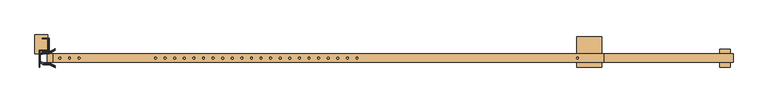
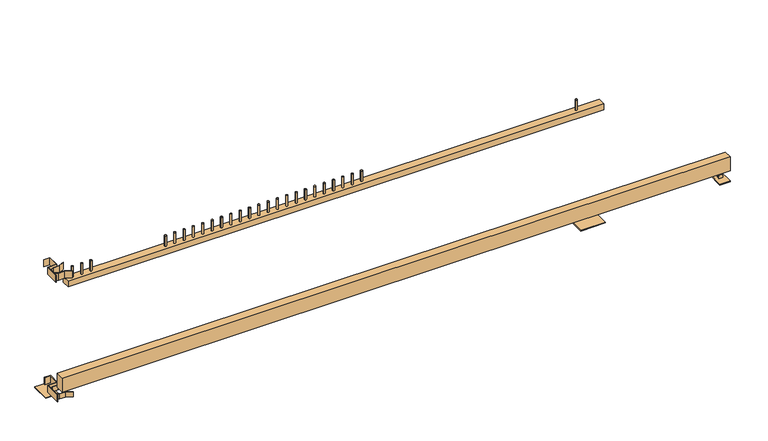
"""IFC4 building model written with IfcOpenShell, lengths in millimetres: door geometry, NLRS_90_DO_UN_schuifpoort met spijlen_gen_rsf : schuifpoort automatisch bxh 7000x1800-NP."""

from ifc_helpers import new_model, si_unit, point, frame, frame_2d, origin, origin_with_axes, place, context, project, spatial, polyline, circle_curve, trimmed, segment, composite_curve, outline, extrude, source, transform, mapped, element, save


def door_84a52a24(model_context):
    return source(origin(), model_context, "Body", "SweptSolid", [
        extrude(outline(composite_curve([segment(trimmed(circle_curve(frame_2d((-3115.5, 0.0)), 12.5), [point((-3103.0, 0.0))], [point((-3128.0, 0.0))], False, "CARTESIAN"), True, "CONTINUOUS"), segment(trimmed(circle_curve(frame_2d((-3115.5, 0.0)), 12.5), [point((-3128.0, 0.0))], [point((-3103.0, 0.0))], False, "CARTESIAN"), True, "CONTINUOUS")], self_intersect=False)), frame((0.0, 0.0, 1650.0), z_axis=(0.0, 0.0, 1.0), x_axis=(1.0, 0.0, 0.0)), (0.0, 0.0, 1.0), 150.0),
        extrude(outline(composite_curve([segment(trimmed(circle_curve(frame_2d((-3241.5, 0.0)), 12.5), [point((-3229.0, 0.0))], [point((-3254.0, 0.0))], False, "CARTESIAN"), True, "CONTINUOUS"), segment(trimmed(circle_curve(frame_2d((-3241.5, 0.0)), 12.5), [point((-3254.0, 0.0))], [point((-3229.0, 0.0))], False, "CARTESIAN"), True, "CONTINUOUS")], self_intersect=False)), frame((0.0, 0.0, 1650.0), z_axis=(0.0, 0.0, 1.0), x_axis=(1.0, 0.0, 0.0)), (0.0, 0.0, 1.0), 150.0),
        extrude(outline(composite_curve([segment(trimmed(circle_curve(frame_2d((-3367.5, 0.0)), 12.5), [point((-3355.0, 0.0))], [point((-3380.0, 0.0))], False, "CARTESIAN"), True, "CONTINUOUS"), segment(trimmed(circle_curve(frame_2d((-3367.5, 0.0)), 12.5), [point((-3380.0, 0.0))], [point((-3355.0, 0.0))], False, "CARTESIAN"), True, "CONTINUOUS")], self_intersect=False)), frame((0.0, 0.0, 1650.0), z_axis=(0.0, 0.0, 1.0), x_axis=(1.0, 0.0, 0.0)), (0.0, 0.0, 1.0), 150.0),
        extrude(outline(polyline([(3745.0, 280.5), (3745.0, -119.5), (3415.0, -119.5), (3415.0, 280.5), (3745.0, 280.5)])), origin_with_axes(), (0.0, 0.0, 1.0), 12.0),
        extrude(outline(composite_curve([segment(trimmed(circle_curve(frame_2d((3424.5, 0.0)), 12.5), [point((3437.0, 0.0))], [point((3412.0, 0.0))], False, "CARTESIAN"), True, "CONTINUOUS"), segment(trimmed(circle_curve(frame_2d((3424.5, 0.0)), 12.5), [point((3412.0, 0.0))], [point((3437.0, 0.0))], False, "CARTESIAN"), True, "CONTINUOUS")], self_intersect=False)), frame((0.0, 0.0, 1650.0), z_axis=(0.0, 0.0, 1.0), x_axis=(1.0, 0.0, 0.0)), (0.0, 0.0, 1.0), 150.0),
        extrude(outline(composite_curve([segment(trimmed(circle_curve(frame_2d((-727.5, 0.0)), 12.5), [point((-715.0, 0.0))], [point((-740.0, 0.0))], False, "CARTESIAN"), True, "CONTINUOUS"), segment(trimmed(circle_curve(frame_2d((-727.5, 0.0)), 12.5), [point((-740.0, 0.0))], [point((-715.0, 0.0))], False, "CARTESIAN"), True, "CONTINUOUS")], self_intersect=False)), frame((0.0, 0.0, 1650.0), z_axis=(0.0, 0.0, 1.0), x_axis=(1.0, 0.0, 0.0)), (0.0, 0.0, 1.0), 150.0),
        extrude(outline(composite_curve([segment(trimmed(circle_curve(frame_2d((-2111.5, 0.0)), 12.5), [point((-2099.0, 0.0))], [point((-2124.0, 0.0))], False, "CARTESIAN"), True, "CONTINUOUS"), segment(trimmed(circle_curve(frame_2d((-2111.5, 0.0)), 12.5), [point((-2124.0, 0.0))], [point((-2099.0, 0.0))], False, "CARTESIAN"), True, "CONTINUOUS")], self_intersect=False)), frame((0.0, 0.0, 1650.0), z_axis=(0.0, 0.0, 1.0), x_axis=(1.0, 0.0, 0.0)), (0.0, 0.0, 1.0), 150.0),
        extrude(outline(composite_curve([segment(trimmed(circle_curve(frame_2d((531.5, 0.0)), 12.5), [point((544.0, 0.0))], [point((519.0, 0.0))], False, "CARTESIAN"), True, "CONTINUOUS"), segment(trimmed(circle_curve(frame_2d((531.5, 0.0)), 12.5), [point((519.0, 0.0))], [point((544.0, 0.0))], False, "CARTESIAN"), True, "CONTINUOUS")], self_intersect=False)), frame((0.0, 0.0, 1650.0), z_axis=(0.0, 0.0, 1.0), x_axis=(1.0, 0.0, 0.0)), (0.0, 0.0, 1.0), 150.0),
        extrude(outline(composite_curve([segment(trimmed(circle_curve(frame_2d((405.5, 0.0)), 12.5), [point((418.0, 0.0))], [point((393.0, 0.0))], False, "CARTESIAN"), True, "CONTINUOUS"), segment(trimmed(circle_curve(frame_2d((405.5, 0.0)), 12.5), [point((393.0, 0.0))], [point((418.0, 0.0))], False, "CARTESIAN"), True, "CONTINUOUS")], self_intersect=False)), frame((0.0, 0.0, 1650.0), z_axis=(0.0, 0.0, 1.0), x_axis=(1.0, 0.0, 0.0)), (0.0, 0.0, 1.0), 150.0),
        extrude(outline(composite_curve([segment(trimmed(circle_curve(frame_2d((279.5, 0.0)), 12.5), [point((292.0, 0.0))], [point((267.0, 0.0))], False, "CARTESIAN"), True, "CONTINUOUS"), segment(trimmed(circle_curve(frame_2d((279.5, 0.0)), 12.5), [point((267.0, 0.0))], [point((292.0, 0.0))], False, "CARTESIAN"), True, "CONTINUOUS")], self_intersect=False)), frame((0.0, 0.0, 1650.0), z_axis=(0.0, 0.0, 1.0), x_axis=(1.0, 0.0, 0.0)), (0.0, 0.0, 1.0), 150.0),
        extrude(outline(composite_curve([segment(trimmed(circle_curve(frame_2d((153.5, 0.0)), 12.5), [point((166.0, 0.0))], [point((141.0, 0.0))], False, "CARTESIAN"), True, "CONTINUOUS"), segment(trimmed(circle_curve(frame_2d((153.5, 0.0)), 12.5), [point((141.0, 0.0))], [point((166.0, 0.0))], False, "CARTESIAN"), True, "CONTINUOUS")], self_intersect=False)), frame((0.0, 0.0, 1650.0), z_axis=(0.0, 0.0, 1.0), x_axis=(1.0, 0.0, 0.0)), (0.0, 0.0, 1.0), 150.0),
        extrude(outline(composite_curve([segment(trimmed(circle_curve(frame_2d((27.5, 0.0)), 12.5), [point((40.0, 0.0))], [point((15.0, 0.0))], False, "CARTESIAN"), True, "CONTINUOUS"), segment(trimmed(circle_curve(frame_2d((27.5, 0.0)), 12.5), [point((15.0, 0.0))], [point((40.0, 0.0))], False, "CARTESIAN"), True, "CONTINUOUS")], self_intersect=False)), frame((0.0, 0.0, 1650.0), z_axis=(0.0, 0.0, 1.0), x_axis=(1.0, 0.0, 0.0)), (0.0, 0.0, 1.0), 150.0),
        extrude(outline(composite_curve([segment(trimmed(circle_curve(frame_2d((-98.5, 0.0)), 12.5), [point((-86.0, 0.0))], [point((-111.0, 0.0))], False, "CARTESIAN"), True, "CONTINUOUS"), segment(trimmed(circle_curve(frame_2d((-98.5, 0.0)), 12.5), [point((-111.0, 0.0))], [point((-86.0, 0.0))], False, "CARTESIAN"), True, "CONTINUOUS")], self_intersect=False)), frame((0.0, 0.0, 1650.0), z_axis=(0.0, 0.0, 1.0), x_axis=(1.0, 0.0, 0.0)), (0.0, 0.0, 1.0), 150.0),
        extrude(outline(composite_curve([segment(trimmed(circle_curve(frame_2d((-224.5, 0.0)), 12.5), [point((-212.0, 0.0))], [point((-237.0, 0.0))], False, "CARTESIAN"), True, "CONTINUOUS"), segment(trimmed(circle_curve(frame_2d((-224.5, 0.0)), 12.5), [point((-237.0, 0.0))], [point((-212.0, 0.0))], False, "CARTESIAN"), True, "CONTINUOUS")], self_intersect=False)), frame((0.0, 0.0, 1650.0), z_axis=(0.0, 0.0, 1.0), x_axis=(1.0, 0.0, 0.0)), (0.0, 0.0, 1.0), 150.0),
        extrude(outline(composite_curve([segment(trimmed(circle_curve(frame_2d((-350.5, 0.0)), 12.5), [point((-338.0, 0.0))], [point((-363.0, 0.0))], False, "CARTESIAN"), True, "CONTINUOUS"), segment(trimmed(circle_curve(frame_2d((-350.5, 0.0)), 12.5), [point((-363.0, 0.0))], [point((-338.0, 0.0))], False, "CARTESIAN"), True, "CONTINUOUS")], self_intersect=False)), frame((0.0, 0.0, 1650.0), z_axis=(0.0, 0.0, 1.0), x_axis=(1.0, 0.0, 0.0)), (0.0, 0.0, 1.0), 150.0),
        extrude(outline(composite_curve([segment(trimmed(circle_curve(frame_2d((-476.5, 0.0)), 12.5), [point((-464.0, 0.0))], [point((-489.0, 0.0))], False, "CARTESIAN"), True, "CONTINUOUS"), segment(trimmed(circle_curve(frame_2d((-476.5, 0.0)), 12.5), [point((-489.0, 0.0))], [point((-464.0, 0.0))], False, "CARTESIAN"), True, "CONTINUOUS")], self_intersect=False)), frame((0.0, 0.0, 1650.0), z_axis=(0.0, 0.0, 1.0), x_axis=(1.0, 0.0, 0.0)), (0.0, 0.0, 1.0), 150.0),
        extrude(outline(composite_curve([segment(trimmed(circle_curve(frame_2d((-602.5, 0.0)), 12.5), [point((-590.0, 0.0))], [point((-615.0, 0.0))], False, "CARTESIAN"), True, "CONTINUOUS"), segment(trimmed(circle_curve(frame_2d((-602.5, 0.0)), 12.5), [point((-615.0, 0.0))], [point((-590.0, 0.0))], False, "CARTESIAN"), True, "CONTINUOUS")], self_intersect=False)), frame((0.0, 0.0, 1650.0), z_axis=(0.0, 0.0, 1.0), x_axis=(1.0, 0.0, 0.0)), (0.0, 0.0, 1.0), 150.0),
        extrude(outline(composite_curve([segment(trimmed(circle_curve(frame_2d((-852.5, 0.0)), 12.5), [point((-840.0, 0.0))], [point((-865.0, 0.0))], False, "CARTESIAN"), True, "CONTINUOUS"), segment(trimmed(circle_curve(frame_2d((-852.5, 0.0)), 12.5), [point((-865.0, 0.0))], [point((-840.0, 0.0))], False, "CARTESIAN"), True, "CONTINUOUS")], self_intersect=False)), frame((0.0, 0.0, 1650.0), z_axis=(0.0, 0.0, 1.0), x_axis=(1.0, 0.0, 0.0)), (0.0, 0.0, 1.0), 150.0),
        extrude(outline(composite_curve([segment(trimmed(circle_curve(frame_2d((-978.5, 0.0)), 12.5), [point((-966.0, 0.0))], [point((-991.0, 0.0))], False, "CARTESIAN"), True, "CONTINUOUS"), segment(trimmed(circle_curve(frame_2d((-978.5, 0.0)), 12.5), [point((-991.0, 0.0))], [point((-966.0, 0.0))], False, "CARTESIAN"), True, "CONTINUOUS")], self_intersect=False)), frame((0.0, 0.0, 1650.0), z_axis=(0.0, 0.0, 1.0), x_axis=(1.0, 0.0, 0.0)), (0.0, 0.0, 1.0), 150.0),
        extrude(outline(composite_curve([segment(trimmed(circle_curve(frame_2d((-1104.5, 0.0)), 12.5), [point((-1092.0, 0.0))], [point((-1117.0, 0.0))], False, "CARTESIAN"), True, "CONTINUOUS"), segment(trimmed(circle_curve(frame_2d((-1104.5, 0.0)), 12.5), [point((-1117.0, 0.0))], [point((-1092.0, 0.0))], False, "CARTESIAN"), True, "CONTINUOUS")], self_intersect=False)), frame((0.0, 0.0, 1650.0), z_axis=(0.0, 0.0, 1.0), x_axis=(1.0, 0.0, 0.0)), (0.0, 0.0, 1.0), 150.0),
        extrude(outline(composite_curve([segment(trimmed(circle_curve(frame_2d((-1230.5, 0.0)), 12.5), [point((-1218.0, 0.0))], [point((-1243.0, 0.0))], False, "CARTESIAN"), True, "CONTINUOUS"), segment(trimmed(circle_curve(frame_2d((-1230.5, 0.0)), 12.5), [point((-1243.0, 0.0))], [point((-1218.0, 0.0))], False, "CARTESIAN"), True, "CONTINUOUS")], self_intersect=False)), frame((0.0, 0.0, 1650.0), z_axis=(0.0, 0.0, 1.0), x_axis=(1.0, 0.0, 0.0)), (0.0, 0.0, 1.0), 150.0),
        extrude(outline(composite_curve([segment(trimmed(circle_curve(frame_2d((-1356.5, 0.0)), 12.5), [point((-1344.0, 0.0))], [point((-1369.0, 0.0))], False, "CARTESIAN"), True, "CONTINUOUS"), segment(trimmed(circle_curve(frame_2d((-1356.5, 0.0)), 12.5), [point((-1369.0, 0.0))], [point((-1344.0, 0.0))], False, "CARTESIAN"), True, "CONTINUOUS")], self_intersect=False)), frame((0.0, 0.0, 1650.0), z_axis=(0.0, 0.0, 1.0), x_axis=(1.0, 0.0, 0.0)), (0.0, 0.0, 1.0), 150.0),
        extrude(outline(composite_curve([segment(trimmed(circle_curve(frame_2d((-1482.5, 0.0)), 12.5), [point((-1470.0, 0.0))], [point((-1495.0, 0.0))], False, "CARTESIAN"), True, "CONTINUOUS"), segment(trimmed(circle_curve(frame_2d((-1482.5, 0.0)), 12.5), [point((-1495.0, 0.0))], [point((-1470.0, 0.0))], False, "CARTESIAN"), True, "CONTINUOUS")], self_intersect=False)), frame((0.0, 0.0, 1650.0), z_axis=(0.0, 0.0, 1.0), x_axis=(1.0, 0.0, 0.0)), (0.0, 0.0, 1.0), 150.0),
        extrude(outline(composite_curve([segment(trimmed(circle_curve(frame_2d((-1608.5, 0.0)), 12.5), [point((-1596.0, 0.0))], [point((-1621.0, 0.0))], False, "CARTESIAN"), True, "CONTINUOUS"), segment(trimmed(circle_curve(frame_2d((-1608.5, 0.0)), 12.5), [point((-1621.0, 0.0))], [point((-1596.0, 0.0))], False, "CARTESIAN"), True, "CONTINUOUS")], self_intersect=False)), frame((0.0, 0.0, 1650.0), z_axis=(0.0, 0.0, 1.0), x_axis=(1.0, 0.0, 0.0)), (0.0, 0.0, 1.0), 150.0),
        extrude(outline(composite_curve([segment(trimmed(circle_curve(frame_2d((-1734.5, 0.0)), 12.5), [point((-1722.0, 0.0))], [point((-1747.0, 0.0))], False, "CARTESIAN"), True, "CONTINUOUS"), segment(trimmed(circle_curve(frame_2d((-1734.5, 0.0)), 12.5), [point((-1747.0, 0.0))], [point((-1722.0, 0.0))], False, "CARTESIAN"), True, "CONTINUOUS")], self_intersect=False)), frame((0.0, 0.0, 1650.0), z_axis=(0.0, 0.0, 1.0), x_axis=(1.0, 0.0, 0.0)), (0.0, 0.0, 1.0), 150.0),
        extrude(outline(composite_curve([segment(trimmed(circle_curve(frame_2d((-1860.5, 0.0)), 12.5), [point((-1848.0, 0.0))], [point((-1873.0, 0.0))], False, "CARTESIAN"), True, "CONTINUOUS"), segment(trimmed(circle_curve(frame_2d((-1860.5, 0.0)), 12.5), [point((-1873.0, 0.0))], [point((-1848.0, 0.0))], False, "CARTESIAN"), True, "CONTINUOUS")], self_intersect=False)), frame((0.0, 0.0, 1650.0), z_axis=(0.0, 0.0, 1.0), x_axis=(1.0, 0.0, 0.0)), (0.0, 0.0, 1.0), 150.0),
        extrude(outline(composite_curve([segment(trimmed(circle_curve(frame_2d((-1986.5, 0.0)), 12.5), [point((-1974.0, 0.0))], [point((-1999.0, 0.0))], False, "CARTESIAN"), True, "CONTINUOUS"), segment(trimmed(circle_curve(frame_2d((-1986.5, 0.0)), 12.5), [point((-1999.0, 0.0))], [point((-1974.0, 0.0))], False, "CARTESIAN"), True, "CONTINUOUS")], self_intersect=False)), frame((0.0, 0.0, 1650.0), z_axis=(0.0, 0.0, 1.0), x_axis=(1.0, 0.0, 0.0)), (0.0, 0.0, 1.0), 150.0),
        extrude(outline(polyline([(-3430.0, -104.7285156), (-3510.75, -63.3066406), (-3586.53125, -63.3066406), (-3633.0, -39.4667969), (-3633.0, 39.4707031), (-3586.53125, 63.3105469), (-3510.75, 63.3105469), (-3430.0, 104.7324219), (-3428.15625, 101.1738281), (-3509.78125, 59.3105469), (-3585.5625, 59.3105469), (-3629.0, 37.0332031), (-3629.0, -37.0292969), (-3585.5625, -59.3066406), (-3509.78125, -59.3066406), (-3428.15625, -101.1699219), (-3430.0, -104.7285156)])), frame((0.0, 0.0, 1720.0), z_axis=(0.0, 0.0, 1.0), x_axis=(1.0, 0.0, 0.0)), (0.0, 0.0, 1.0), 100.0),
        extrude(outline(polyline([(-3638.0, 105.534128), (-3524.015625, 105.534128), (-3524.015625, 255.534128), (-3601.25, 255.534128), (-3601.25, 260.534128), (-3519.015625, 260.534128), (-3519.015625, 100.534128), (-3633.0, 100.534128), (-3633.0, -85.4980469), (-3638.0, -85.4980469), (-3638.0, 105.534128)])), frame((0.0, 0.0, 1720.0), z_axis=(0.0, 0.0, 1.0), x_axis=(1.0, 0.0, 0.0)), (0.0, 0.0, 1.0), 100.0),
        extrude(outline(composite_curve([segment(polyline([(12.0, 5337.0), (12.0, 5387.0), (42.0, 5387.0)]), True, "CONTINUOUS"), segment(trimmed(circle_curve(frame_2d((42.0, 5362.0)), 25.0), [point((42.0, 5387.0))], [point((42.0, 5337.0))], False, "CARTESIAN"), True, "CONTINUOUS"), segment(polyline([(42.0, 5337.0), (12.0, 5337.0)]), True, "CONTINUOUS")], self_intersect=False)), frame((0.0, 11.0, 0.0), z_axis=(0.0, 1.0, 0.0), x_axis=(0.0, 0.0, 1.0)), (0.0, 0.0, 1.0), 8.0),
        extrude(outline(composite_curve([segment(polyline([(12.0, 5337.0), (12.0, 5387.0), (42.0, 5387.0)]), True, "CONTINUOUS"), segment(trimmed(circle_curve(frame_2d((42.0, 5362.0)), 25.0), [point((42.0, 5387.0))], [point((42.0, 5337.0))], False, "CARTESIAN"), True, "CONTINUOUS"), segment(polyline([(42.0, 5337.0), (12.0, 5337.0)]), True, "CONTINUOUS")], self_intersect=False)), frame((0.0, -19.0, 0.0), z_axis=(0.0, 1.0, 0.0), x_axis=(0.0, 0.0, 1.0)), (0.0, 0.0, 1.0), 8.0),
        extrude(outline(polyline([(5432.0, 120.0), (5432.0, -120.0), (5292.0, -120.0), (5292.0, 120.0), (5432.0, 120.0)])), origin_with_axes(), (0.0, 0.0, 1.0), 12.0),
        extrude(outline(polyline([(5372.0, 11.0), (5372.0, -11.0), (5352.0, -11.0), (5352.0, 11.0), (5372.0, 11.0)])), frame((0.0, 0.0, 12.0), z_axis=(0.0, 0.0, 1.0), x_axis=(1.0, 0.0, 0.0)), (0.0, 0.0, 1.0), 88.0),
        extrude(outline(polyline([(-3429.5, -126.125), (-3509.75, -84.8125), (-3585.75, -84.8125), (-3633.0, -60.585938), (-3633.0, 60.585938), (-3585.75, 84.8125), (-3509.75, 84.8125), (-3429.5, 126.125), (-3427.2114608, 121.6794867), (-3508.5385575, 79.8125), (-3584.542883, 79.8125), (-3628.0, 57.5306685), (-3628.0, -57.5306685), (-3584.542883, -79.8125), (-3508.5385575, -79.8125), (-3427.2114608, -121.6794867), (-3429.5, -126.125)])), frame((0.0, 0.0, 39.0), z_axis=(0.0, 0.0, 1.0), x_axis=(1.0, 0.0, 0.0)), (0.0, 0.0, 1.0), 70.0),
        extrude(outline(polyline([(-3638.0, 105.5), (-3515.0, 105.5), (-3515.0, 255.5), (-3593.0, 255.5), (-3593.0, 260.5), (-3510.0, 260.5), (-3510.0, 100.5), (-3633.0, 100.5), (-3633.0, -119.5), (-3638.0, -119.5), (-3638.0, 105.5)])), frame((0.0, 0.0, 39.0), z_axis=(0.0, 0.0, 1.0), x_axis=(1.0, 0.0, 0.0)), (0.0, 0.0, 1.0), 100.0),
        extrude(outline(polyline([(5467.0, 55.0), (5467.0, -55.0), (-3535.5, -55.0), (-3535.5, 55.0), (5467.0, 55.0)])), frame((0.0, 0.0, 100.0), z_axis=(0.0, 0.0, 1.0), x_axis=(1.0, 0.0, 0.0)), (0.0, 0.0, 1.0), 200.0),
        extrude(outline(polyline([(-3525.0, 305.0), (-3525.0, 55.0), (-3695.0, 55.0), (-3695.0, 305.0), (-3525.0, 305.0)])), origin_with_axes(), (0.0, 0.0, 1.0), 12.0),
        extrude(outline(polyline([(3767.5, 55.0), (3767.5, -55.0), (-3455.5, -55.0), (-3455.5, 55.0), (3767.5, 55.0)])), frame((0.0, 0.0, 1570.0), z_axis=(0.0, 0.0, 1.0), x_axis=(1.0, 0.0, 0.0)), (0.0, 0.0, 1.0), 80.0),
    ])


if __name__ == "__main__":
    model = new_model("IFC4")
    model_context = context("Model", 3, world=origin())
    ifc_project = project(units=[si_unit("LENGTHUNIT", "METRE", prefix="MILLI")], contexts=[model_context])
    site = spatial("IfcSite", under=ifc_project)
    building = spatial("IfcBuilding", under=site)
    placement = place(None, origin())
    door_shape = door_84a52a24(model_context)
    element("IfcDoor", 1, ObjectType="NLRS_90_DO_UN_schuifpoort met spijlen_gen_rsf : schuifpoort automatisch bxh 7000x1800-NP", at=placement, inside=building, context=model_context, shape_type="MappedRepresentation", body=[
        mapped(door_shape, transform((0.0, 0.0, 0.0), x_axis=(1.0, 0.0, 0.0), y_axis=(0.0, 1.0, 0.0), z_axis=(0.0, 0.0, 1.0))),
    ])
    save(model, "model.ifc")

# Revit data of these elements
# Type "NLRS_90_DO_UN_schuifpoort met spijlen_gen_rsf : schuifpoort automatisch bxh 7000x1800-NP"
#   Type IFC Predefined Type = "GATE"
#   Export Type to IFC As = "IfcDoorType"
#   Type IfcGUID = "1A81voHkv98RYujw6ZYnX6"
#   IfcName[Type] = "schuifpoort automatisch bxh 7000x1800-NP"
#   IfcDescription[Type] = "schuifpoort doorgang bxh 7000x1800mm"
#   NLRS_C_revit_versie = ""
#   NLRS_C_omschrijving_03 [instance default] = "doorgangsmaat"
#   NLRS_C_omschrijving_02 [instance default] = "stootplaat"
#   NLRS_C_omschrijving_01 [instance default] = "rolpoort"
#   NLRS_C_content_versie = ""
#   NLRS_C_content_provider = ""
#   NLRS_C_content_handleiding = ""
#   NLRS_C_content_datum_uitgifte = ""
#   NLRS_C_content_datum_gewijzigd = ""
#   NLRS_C_content_creator = ""
#   Model = "generiek"
#   Manufacturer = "Revit Standards Foundation"
#   Description = "schuifpoort doorgang bxh 7000x1800mm"
#   Assembly Code = "90.32"
#   NLRS_C_hoogte = 1800.00 mm
#   NLRS_C_breedte_03 = 7000.00 mm
#   NLRS_C_materiaal_02 = NLRS_n5_rubber_gen_bf
#   NLRS_C_materiaal_01 = NLRS_h4_aluminium 250-255-255_gen_rsf
#   URL = ""
#   Keynote = ""
#   Default Elevation = 0
# Element 1 (IfcDoor, "NLRS_90_DO_UN_schuifpoort met spijlen_gen_rsf : schuifpoort automatisch bxh 7000x1800-NP")
#   Materials on its faces: "NLRS_h4_aluminium 250-255-255_gen_rsf", "NLRS_n5_rubber_gen_bf"
# Materials
#   "NLRS_n5_rubber_gen_bf": class "N - Kunststoffen, rubbers", colour RGB 63 63 63, transparency 0, Keynote = "n5", Model = "generiek", Manufacturer = "Revit Standards Foundation", URL = "www.revitstandards.org", Description = "rubber daktegels 600x600mm", Cost = 0
#   "NLRS_h4_aluminium 250-255-255_gen_rsf": class "BCB class", colour RGB 250 255 255, transparency 0, Keynote = "h4", Model = "generiek", Manufacturer = "Revit Standards Foundation", URL = "www.revitstandards.org", Description = "aluminium wit", Cost = 0
